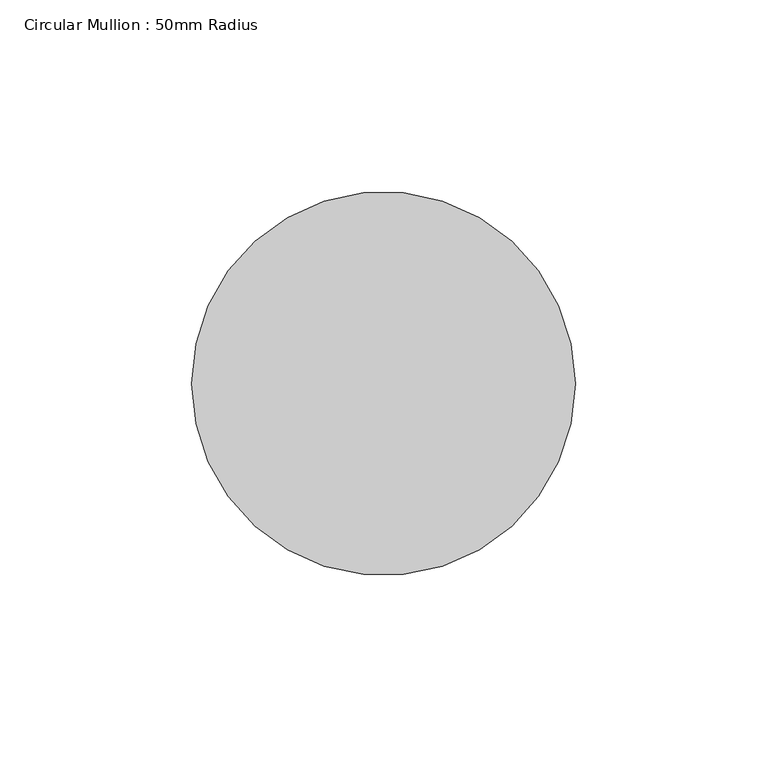
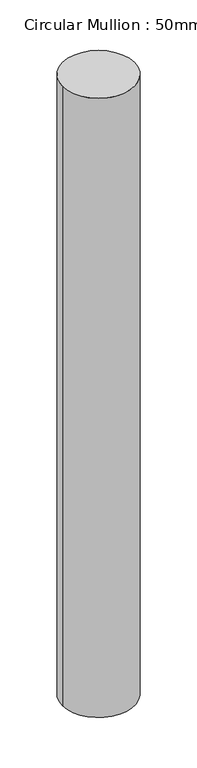
"""IFC4 building model written with IfcOpenShell, lengths in millimetres: member geometry, Circular Mullion : 50mm Radius."""

from ifc_helpers import new_model, si_unit, point, frame, origin, origin_2d, place, context, project, spatial, circle_curve, trimmed, segment, composite_curve, outline, extrude, source, transform, mapped, element, save


def circular_mullion_50mm_radius_afbc9d9e(model_context):
    return source(origin(), model_context, "Body", "SweptSolid", [
        extrude(outline(composite_curve([segment(trimmed(circle_curve(origin_2d(), 50.0), [point((50.0, 0.0))], [point((-50.0, 0.0))], False, "CARTESIAN"), True, "CONTINUOUS"), segment(trimmed(circle_curve(origin_2d(), 50.0), [point((-50.0, 0.0))], [point((50.0, 0.0))], False, "CARTESIAN"), True, "CONTINUOUS")], self_intersect=False)), frame((0.0, 0.0, -906.1359203), z_axis=(0.0, 0.0, 1.0), x_axis=(1.0, 0.0, 0.0)), (0.0, 0.0, 1.0), 906.1359203),
    ])


if __name__ == "__main__":
    model = new_model("IFC4")
    model_context = context("Model", 3, world=origin())
    ifc_project = project(units=[si_unit("LENGTHUNIT", "METRE", prefix="MILLI")], contexts=[model_context])
    site = spatial("IfcSite", under=ifc_project)
    building = spatial("IfcBuilding", under=site)
    placement = place(None, origin())
    circular_mullion_50mm_radius_shape = circular_mullion_50mm_radius_afbc9d9e(model_context)
    element("IfcMember", 1, ObjectType="Circular Mullion : 50mm Radius", at=placement, inside=building, context=model_context, shape_type="MappedRepresentation", body=[
        mapped(circular_mullion_50mm_radius_shape, transform((0.0, 0.0, 0.0), x_axis=(1.0, 0.0, 0.0), y_axis=(0.0, 1.0, 0.0), z_axis=(0.0, 0.0, 1.0))),
    ])
    save(model, "model.ifc")

# Revit data of these elements
# Type "Circular Mullion : 50mm Radius"
#   built-in parameter 1007350 = 0.164042 (stored number, unit not read)
# Element 1 (IfcMember, "Circular Mullion : 50mm Radius")
#   Materials on its faces: "Aluminium"
# Materials
#   "Aluminium": class "Metal", colour RGB 247 247 247, transparency 0, Description = "Aluminium 6061", Cost = 0
